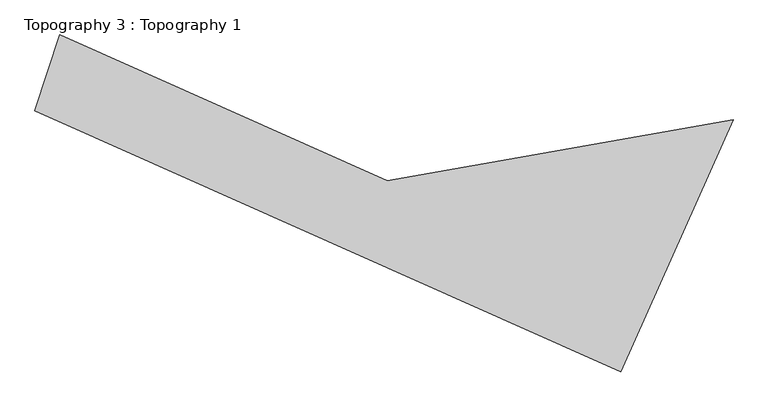
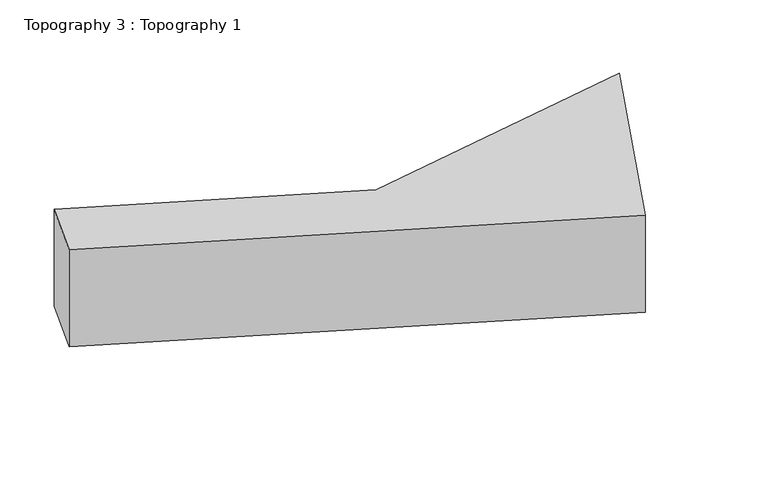
"""IFC4 building model written with IfcOpenShell, lengths in millimetres: proxy geometry, Topography 3 : Topography 1."""

from ifc_helpers import new_model, si_unit, frame, origin, place, context, project, spatial, polyline, outline, extrude, source, transform, mapped, element, save


def topography_3_topography_1_7801e185(model_context):
    return source(origin(), model_context, "Body", "SweptSolid", [
        extrude(outline(polyline([(145309.3047745, 82001.3714516), (146247.9969154, 84890.3688002), (158730.8645012, 79332.6380761), (171896.6644567, 81654.1238309), (167627.2203047, 72064.7952613), (145309.3047745, 82001.3714516)])), frame((0.0, 0.0, -10770.0), z_axis=(0.0, 0.0, 1.0), x_axis=(1.0, 0.0, 0.0)), (0.0, 0.0, 1.0), 4996.5755343),
    ])


if __name__ == "__main__":
    model = new_model("IFC4")
    model_context = context("Model", 3, world=origin())
    ifc_project = project(units=[si_unit("LENGTHUNIT", "METRE", prefix="MILLI")], contexts=[model_context])
    site = spatial("IfcSite", under=ifc_project)
    building = spatial("IfcBuilding", under=site)
    placement = place(None, origin())
    topography_3_topography_1_shape = topography_3_topography_1_7801e185(model_context)
    element("IfcBuildingElementProxy", 1, Name="Topography 3 : Topography 1", ObjectType="Topography 3 : Topography 1", at=placement, inside=building, context=model_context, shape_type="MappedRepresentation", body=[
        mapped(topography_3_topography_1_shape, transform((0.0, 0.0, 0.0), x_axis=(1.0, 0.0, 0.0), y_axis=(0.0, 1.0, 0.0), z_axis=(0.0, 0.0, 1.0))),
    ])
    save(model, "model.ifc")

# Revit data of these elements
# Element 1 (IfcBuildingElementProxy, "Topography 3 : Topography 1")
#   Materials on its faces: "Earth"
# Materials
#   "Earth": class "Generic", colour RGB 97 75 62, transparency 0, Description = "Soil", Cost = 0
